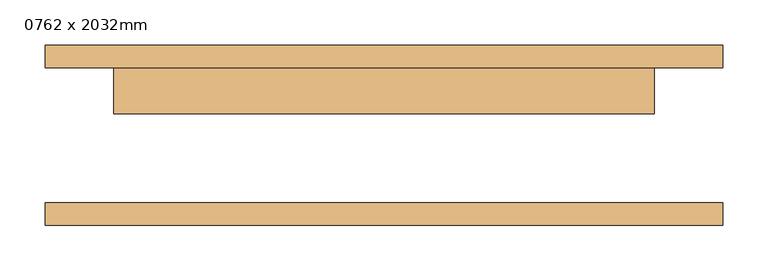
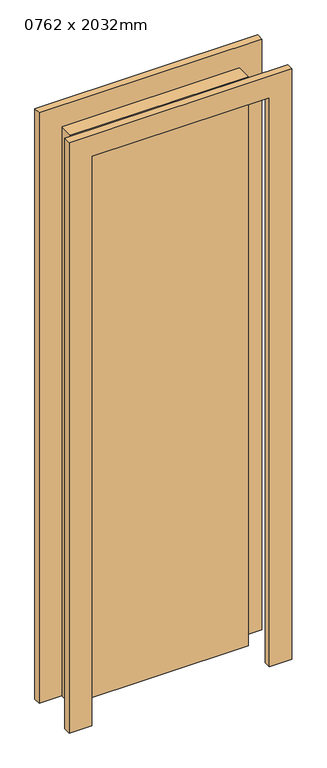
"""IFC4 building model written with IfcOpenShell, lengths in millimetres: door geometry, M_Folha única : 0762 x 2032mm."""

from ifc_helpers import new_model, si_unit, frame, origin, origin_with_axes, place, context, project, spatial, polyline, outline, extrude, source, transform, mapped, element, save


def door_0762_x_2032mm_f712f77f(model_context):
    return source(origin(), model_context, "Body", "SweptSolid", [
        extrude(outline(polyline([(2108.0, -376.0), (0.0, -376.0), (0.0, -300.0), (2032.0, -300.0), (2032.0, 300.0), (0.0, 300.0), (0.0, 376.0), (2108.0, 376.0), (2108.0, -376.0)])), frame((0.0, 75.0, 0.0), z_axis=(0.0, 1.0, 0.0), x_axis=(0.0, 0.0, 1.0)), (0.0, 0.0, 1.0), 25.0),
        extrude(outline(polyline([(2108.0, 376.0), (2108.0, -376.0), (0.0, -376.0), (0.0, -300.0), (2032.0, -300.0), (2032.0, 300.0), (0.0, 300.0), (0.0, 376.0), (2108.0, 376.0)])), frame((0.0, -100.0, 0.0), z_axis=(0.0, 1.0, 0.0), x_axis=(0.0, 0.0, 1.0)), (0.0, 0.0, 1.0), 25.0),
        extrude(outline(polyline([(300.0, 24.0), (-300.0, 24.0), (-300.0, 75.0), (300.0, 75.0), (300.0, 24.0)])), origin_with_axes(), (0.0, 0.0, 1.0), 2032.0),
    ])


if __name__ == "__main__":
    model = new_model("IFC4")
    model_context = context("Model", 3, world=origin())
    ifc_project = project(units=[si_unit("LENGTHUNIT", "METRE", prefix="MILLI")], contexts=[model_context])
    site = spatial("IfcSite", under=ifc_project)
    building = spatial("IfcBuilding", under=site)
    placement = place(None, origin())
    door_0762_x_2032mm_shape = door_0762_x_2032mm_f712f77f(model_context)
    element("IfcDoor", 1, ObjectType="M_Folha única : 0762 x 2032mm", at=placement, inside=building, context=model_context, shape_type="MappedRepresentation", body=[
        mapped(door_0762_x_2032mm_shape, transform((0.0, 0.0, 0.0), x_axis=(1.0, 0.0, 0.0), y_axis=(0.0, 1.0, 0.0), z_axis=(0.0, 0.0, 1.0))),
    ])
    save(model, "model.ifc")

# Revit data of these elements
# Type "M_Folha única : 0762 x 2032mm"
#   Type Mark = "28"
#   Construction Type Id = "MDOOR"
#   Analytic Construction = "Metal"
#   Thickness = 0.051 m
#   Thermal Resistance (R) = 0.270117 (m²·K)/W
#   Heat Transfer Coefficient (U) = 3.7021 W/(m²·K)
#   Height = 2.032 m
#   Projeção da apara externa = 0.025 m
#   Projeção da apara interna = 0.025 m
#   Largura da apara = 0.076 m
#   Width = 0.60 m
#   Define Thermal Properties by = 1
#   Material da porta = Porta - Painel
#   Material da moldura = Porta - Batente
#   Visual Light Transmittance = 0
#   Solar Heat Gain Coefficient = 0
#   Function = (empty or 0)
#   Wall Closure = (empty or 0)
# Element 1 (IfcDoor, "M_Folha única : 0762 x 2032mm")
#   Materials on its faces: "Porta - Batente", "Porta - Painel"
# Materials
#   "Porta - Painel": class "Madeira", colour RGB 210 159 95, transparency 0, Cost = 0
#   "Porta - Batente": class "Diversos", colour RGB 118 70 51, transparency 0, Cost = 0
